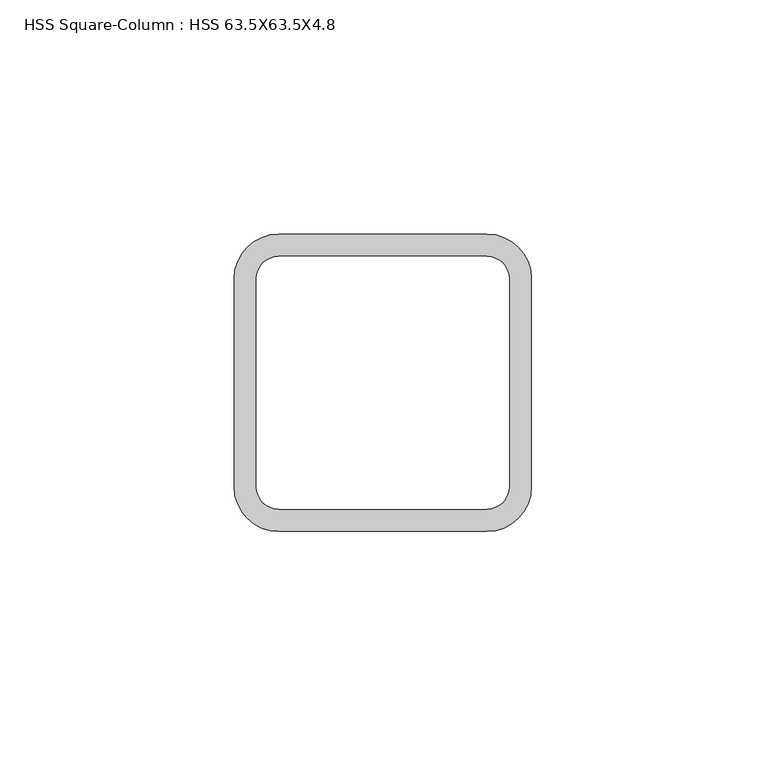
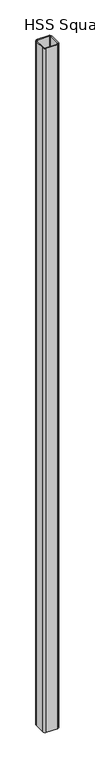
"""IFC4 building model written with IfcOpenShell, lengths in millimetres: column geometry, HSS Square-Column : HSS 63.5X63.5X4.8."""

from ifc_helpers import new_model, si_unit, point, frame, frame_2d, origin, place, context, project, spatial, polyline, circle_curve, trimmed, segment, composite_curve, outline, extrude, source, transform, mapped, element, save


def hss_square_column_hss_63_5x63_5x4_8_fc1831c0(model_context):
    return source(origin(), model_context, "Body", "SweptSolid", [
        extrude(outline(composite_curve([segment(trimmed(circle_curve(frame_2d((22.225, 22.225)), 9.525), [point((22.225, 31.75))], [point((31.75, 22.225))], False, "CARTESIAN"), True, "CONTINUOUS"), segment(polyline([(31.75, 22.225), (31.75, -22.225)]), True, "CONTINUOUS"), segment(trimmed(circle_curve(frame_2d((22.225, -22.225)), 9.525), [point((31.75, -22.225))], [point((22.225, -31.75))], False, "CARTESIAN"), True, "CONTINUOUS"), segment(polyline([(22.225, -31.75), (-22.225, -31.75)]), True, "CONTINUOUS"), segment(trimmed(circle_curve(frame_2d((-22.225, -22.225)), 9.525), [point((-22.225, -31.75))], [point((-31.75, -22.225))], False, "CARTESIAN"), True, "CONTINUOUS"), segment(polyline([(-31.75, -22.225), (-31.75, 22.225)]), True, "CONTINUOUS"), segment(trimmed(circle_curve(frame_2d((-22.225, 22.225)), 9.525), [point((-31.75, 22.225))], [point((-22.225, 31.75))], False, "CARTESIAN"), True, "CONTINUOUS"), segment(polyline([(-22.225, 31.75), (22.225, 31.75)]), True, "CONTINUOUS")], self_intersect=False), holes=[composite_curve([segment(polyline([(22.225, 26.9875), (-22.225, 26.9875)]), True, "CONTINUOUS"), segment(trimmed(circle_curve(frame_2d((-22.225, 22.225)), 4.7625), [point((-22.225, 26.9875))], [point((-26.9875, 22.225))], True, "CARTESIAN"), True, "CONTINUOUS"), segment(polyline([(-26.9875, 22.225), (-26.9875, -22.225)]), True, "CONTINUOUS"), segment(trimmed(circle_curve(frame_2d((-22.225, -22.225)), 4.7625), [point((-26.9875, -22.225))], [point((-22.225, -26.9875))], True, "CARTESIAN"), True, "CONTINUOUS"), segment(polyline([(-22.225, -26.9875), (22.225, -26.9875)]), True, "CONTINUOUS"), segment(trimmed(circle_curve(frame_2d((22.225, -22.225)), 4.7625), [point((22.225, -26.9875))], [point((26.9875, -22.225))], True, "CARTESIAN"), True, "CONTINUOUS"), segment(polyline([(26.9875, -22.225), (26.9875, 22.225)]), True, "CONTINUOUS"), segment(trimmed(circle_curve(frame_2d((22.225, 22.225)), 4.7625), [point((26.9875, 22.225))], [point((22.225, 26.9875))], True, "CARTESIAN"), True, "CONTINUOUS")], self_intersect=False)]), frame((0.0, 0.0, 3220.0), z_axis=(0.0, 0.0, 1.0), x_axis=(1.0, 0.0, 0.0)), (0.0, 0.0, 1.0), 2900.0),
    ])


if __name__ == "__main__":
    model = new_model("IFC4")
    model_context = context("Model", 3, world=origin())
    ifc_project = project(units=[si_unit("LENGTHUNIT", "METRE", prefix="MILLI")], contexts=[model_context])
    site = spatial("IfcSite", under=ifc_project)
    building = spatial("IfcBuilding", under=site)
    placement = place(None, origin())
    hss_square_column_hss_63_5x63_5x4_8_shape = hss_square_column_hss_63_5x63_5x4_8_fc1831c0(model_context)
    element("IfcColumn", 1, ObjectType="HSS Square-Column : HSS 63.5X63.5X4.8", at=placement, inside=building, context=model_context, shape_type="MappedRepresentation", body=[
        mapped(hss_square_column_hss_63_5x63_5x4_8_shape, transform((0.0, 0.0, 0.0), x_axis=(1.0, 0.0, 0.0), y_axis=(0.0, 1.0, 0.0), z_axis=(0.0, 0.0, 1.0))),
    ])
    save(model, "model.ifc")

# Revit data of these elements
# Type "HSS Square-Column : HSS 63.5X63.5X4.8"
#   Section Name Key = "HSS 2 1/2X2 1/2X3/16"
#   Assembly Code = "B10"
#   Width = 6.35 cm
#   Wall Nominal Thickness = 0.4763 cm
#   Wall Design Thickness = 0.442 cm
#   Torsional Moment of Inertia = 93.6521 cm⁴
#   Torsional Modulus = 30.4799 cm³
#   Section Area = 9.93546 cm²
#   Plastic Modulus weak axis = 21.6309 cm³
#   Plastic Modulus strong axis = 21.6309 cm³
#   Outer Fillet = 0.9525 cm
#   Nominal Weight = 8.31884 kgf/m
#   Moment of Inertia weak axis = 56.1912 cm⁴
#   Moment of Inertia strong axis = 56.1912 cm⁴
#   Inner Fillet = 0.4763 cm
#   Height = 6.35 cm
#   Elastic Modulus weak axis = 17.698 cm³
#   Elastic Modulus strong axis = 17.698 cm³
#   Centroid Vertical = 3.175 cm
#   Centroid Horizontal = 3.175 cm
#   Structural Material [instance default] = Steel ASTM A500, Grade B, Rectangular and Square
#   Principal Axes Angle = 0
# Element 1 (IfcColumn, "HSS Square-Column : HSS 63.5X63.5X4.8")
#   Structural Material = none
# Materials
#   "Steel ASTM A500, Grade B, Rectangular and Square": class "Metal", colour RGB 199 199 199, transparency 0, Description = "Carbon steel", Cost = 0
